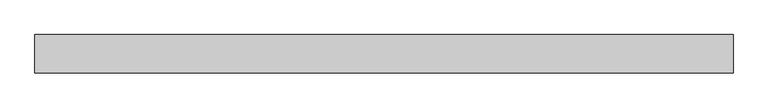
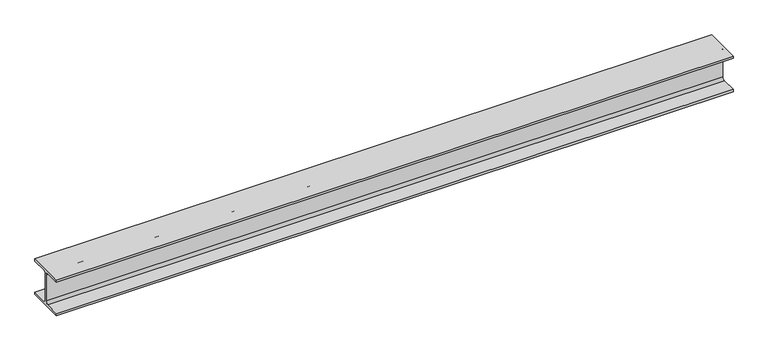
"""IFC4 building model written with IfcOpenShell, lengths in millimetres: beam geometry, 0912_Steel Framing_H-KSD3502 : H_SB_ASB_H-200x200x8x12."""

from ifc_helpers import new_model, si_unit, point, frame, frame_2d, origin, place, context, project, spatial, polyline, circle_curve, trimmed, segment, composite_curve, outline, extrude, source, transform, mapped, element, save


def beam_06b6bcb8(model_context):
    return source(origin(), model_context, "Body", "SweptSolid", [
        extrude(outline(composite_curve([segment(polyline([(100.0, -88.0), (100.0, -100.0), (-100.0, -100.0), (-100.0, -88.0), (-17.0, -88.0)]), True, "CONTINUOUS"), segment(trimmed(circle_curve(frame_2d((-17.0, -75.0)), 13.0), [point((-17.0, -88.0))], [point((-4.0, -75.0))], True, "CARTESIAN"), True, "CONTINUOUS"), segment(polyline([(-4.0, -75.0), (-4.0, 75.0)]), True, "CONTINUOUS"), segment(trimmed(circle_curve(frame_2d((-17.0, 75.0)), 13.0), [point((-4.0, 75.0))], [point((-17.0, 88.0))], True, "CARTESIAN"), True, "CONTINUOUS"), segment(polyline([(-17.0, 88.0), (-100.0, 88.0), (-100.0, 100.0), (100.0, 100.0), (100.0, 88.0), (17.0, 88.0)]), True, "CONTINUOUS"), segment(trimmed(circle_curve(frame_2d((17.0, 75.0)), 13.0), [point((17.0, 88.0))], [point((4.0, 75.0))], True, "CARTESIAN"), True, "CONTINUOUS"), segment(polyline([(4.0, 75.0), (4.0, -75.0)]), True, "CONTINUOUS"), segment(trimmed(circle_curve(frame_2d((17.0, -75.0)), 13.0), [point((4.0, -75.0))], [point((17.0, -88.0))], True, "CARTESIAN"), True, "CONTINUOUS"), segment(polyline([(17.0, -88.0), (100.0, -88.0)]), True, "CONTINUOUS")], self_intersect=False)), frame((-1827.2740995, 0.0, 0.0), z_axis=(1.0, 0.0, 0.0), x_axis=(0.0, 1.0, 0.0)), (0.0, 0.0, 1.0), 3629.4587666),
    ])


if __name__ == "__main__":
    model = new_model("IFC4")
    model_context = context("Model", 3, world=origin())
    ifc_project = project(units=[si_unit("LENGTHUNIT", "METRE", prefix="MILLI")], contexts=[model_context])
    site = spatial("IfcSite", under=ifc_project)
    building = spatial("IfcBuilding", under=site)
    placement = place(None, origin())
    beam_shape = beam_06b6bcb8(model_context)
    element("IfcBeam", 1, ObjectType="0912_Steel Framing_H-KSD3502 : H_SB_ASB_H-200x200x8x12", at=placement, inside=building, context=model_context, shape_type="MappedRepresentation", body=[
        mapped(beam_shape, transform((0.0, 0.0, 0.0), x_axis=(1.0, 0.0, 0.0), y_axis=(0.0, 1.0, 0.0), z_axis=(0.0, 0.0, 1.0))),
    ])
    save(model, "model.ifc")

# Revit data of these elements
# Type "0912_Steel Framing_H-KSD3502 : H_SB_ASB_H-200x200x8x12"
#   H_WM Code_1 = "S01AA002-00001 | Main Steel Structure Fabrication Work | Shelter/Building | Medium Steel - Standard (90KG/M>Weight≥30KG/M) | Material: (   )"
#   H_WM Code_2 = "S03AA028-00001 | Main Steel Structure Erection Work | Shelter/Building | Medium Steel (90KG/M>Weight≥30KG/M) | Material: (   )"
#   H_WM Code_3 = "S01AA010-00001 | Main Steel Structure Fabrication Work | Shelter/Building | Steel Painting/Coating | for Non-Fireproofed Steel Surface, Surface Preparation, Primer, Second & Final Coat | Material: (   )"
#   H_Q'ty Cal Type Tag = "SB-Q2"
#   Width = 20.0 cm
#   Web Thickness = 0.8 cm
#   Web Fillet = 1.3 cm
#   Warping Constant = 141000.0 cm⁶
#   W = 0
#   Torsional Moment of Inertia = 26.2485 cm⁴
#   Section Area = 63.53 cm²
#   Plastic Modulus weak axis = 244.0 cm³
#   Plastic Modulus strong axis = 525.0 cm³
#   Perimeter = 1.16 m²/m
#   Nominal Weight = 49.90 kgf/m
#   Moment of Inertia weak axis = 1600.00 cm⁴
#   Moment of Inertia strong axis = 4720.00 cm⁴
#   Height = 20.0 cm
#   Flange Thickness = 1.2 cm
#   Elastic Modulus weak axis = 160.0 cm³
#   Elastic Modulus strong axis = 472.0 cm³
#   Centroid Vertical = 10.0 cm
#   Centroid Horizontal = 10.0 cm
#   Ix = 47200000
#   Length [instance default] = 1.5240 m
#   Zx = 525000
#   b = 0.2000 m
#   h = 0.2000 m
#   r = 0.0130 m
#   s = 0.0080 m
#   t = 0.0120 m
#   A = 0.006353 m²
#   Structural Material [instance default] = Steel, 45-345
#   Assembly Code = ""
# Element 1 (IfcBeam, "0912_Steel Framing_H-KSD3502 : H_SB_ASB_H-200x200x8x12")
#   Structural Material = none
# Materials
#   "Steel, 45-345": class "Metal", colour RGB 189 187 185, transparency 0, Description = "Steel 345 MPa", Cost = 0
